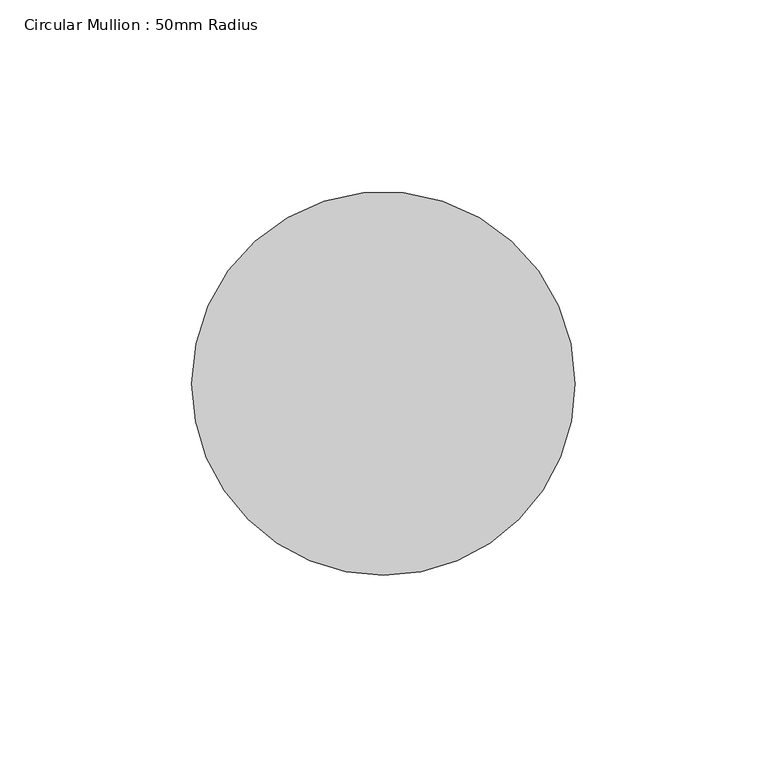
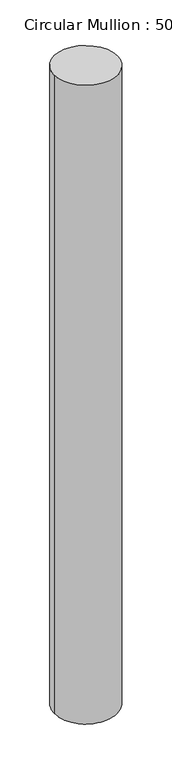
"""IFC4 building model written with IfcOpenShell, lengths in millimetres: member geometry, Circular Mullion : 50mm Radius."""

from ifc_helpers import new_model, si_unit, frame, origin, place, context, project, spatial, ellipse_curve, source, transform, mapped, element, save
from ifc_brep_helpers import plane_surface, cylinder_surface, advanced_brep


def circular_mullion_50mm_radius_f4b702f6(model_context):
    return source(origin(), model_context, "Body", "AdvancedBrep", [
        advanced_brep(
        [(-100.0, 0.0, 1.9077681), (0.0, 0.0, 0.0), (0.0, 0.0, -1070.3892709), (-100.0, 0.0, -1072.2218507)],
        [
            (0, 1, ellipse_curve(frame((-50.0, 0.0, 0.9538841), z_axis=(-0.01906973038879961, -0.021671918604249926, -0.9995832498230997), x_axis=(-0.6603221741338531, -0.750427411329071, 0.028867398100466284)), 50.0208462, 50.0)),
            (1, 2),
            (2, 3, ellipse_curve(frame((-50.0, 0.0, -1071.3055608), z_axis=(-0.018318750336351528, -0.02081846245997146, 0.9996154335577845), x_axis=(0.6603434346278121, 0.750451572955152, 0.027730578664756464)), 50.0192357, 50.0)),
            (3, 0),
            (1, 0, ellipse_curve(frame((-50.0, 0.0, 0.9538841), z_axis=(-0.01906973038879961, -0.021671918604249926, -0.9995832498230997), x_axis=(-0.6603221741338531, -0.750427411329071, 0.028867398100466284)), 50.0208462, 50.0)),
            (3, 2, ellipse_curve(frame((-50.0, 0.0, -1071.3055608), z_axis=(-0.018318750336351528, -0.02081846245997146, 0.9996154335577845), x_axis=(0.6603434346278121, 0.750451572955152, 0.027730578664756464)), 50.0192357, 50.0)),
        ],
        [
            cylinder_surface(frame((-50.0, 0.0, 0.0), z_axis=(0.0, 0.0, 1.0), x_axis=(1.0, 0.0, 0.0)), 50.0),
            plane_surface(frame((-228.8256381, 201.3501114, 0.0), z_axis=(0.01906973038879961, 0.021671918604249926, 0.9995832498230997), x_axis=(0.6603221741338544, 0.7504274113290698, -0.02886739810046519))),
            plane_surface(frame((-228.8256381, 201.3501114, -1070.3892709), z_axis=(0.018318750336351528, 0.02081846245997146, -0.9996154335577845), x_axis=(0.660343434627812, 0.7504515729551521, 0.027730578664766806))),
        ],
        [
            (0, [[1, 2, 3, 4]]),
            (0, [[5, -4, 6, -2]]),
            (1, [[-1, -5]]),
            (2, [[-6, -3]]),
        ],
    ),
    ])


if __name__ == "__main__":
    model = new_model("IFC4")
    model_context = context("Model", 3, world=origin())
    ifc_project = project(units=[si_unit("LENGTHUNIT", "METRE", prefix="MILLI")], contexts=[model_context])
    site = spatial("IfcSite", under=ifc_project)
    building = spatial("IfcBuilding", under=site)
    placement = place(None, origin())
    circular_mullion_50mm_radius_shape = circular_mullion_50mm_radius_f4b702f6(model_context)
    element("IfcMember", 1, ObjectType="Circular Mullion : 50mm Radius", at=placement, inside=building, context=model_context, shape_type="MappedRepresentation", body=[
        mapped(circular_mullion_50mm_radius_shape, transform((0.0, 0.0, 0.0), x_axis=(1.0, 0.0, 0.0), y_axis=(0.0, 1.0, 0.0), z_axis=(0.0, 0.0, 1.0))),
    ])
    save(model, "model.ifc")

# Revit data of these elements
# Type "Circular Mullion : 50mm Radius"
#   built-in parameter 1007350 = 0.164042 (stored number, unit not read)
# Element 1 (IfcMember, "Circular Mullion : 50mm Radius")
#   Materials on its faces: "Aluminium"
# Materials
#   "Aluminium": class "Metal", colour RGB 247 247 247, transparency 0, Description = "Aluminium 6061", Cost = 0
